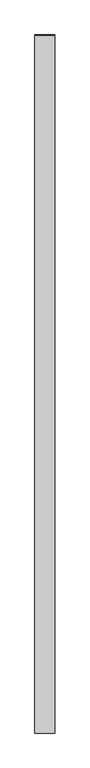
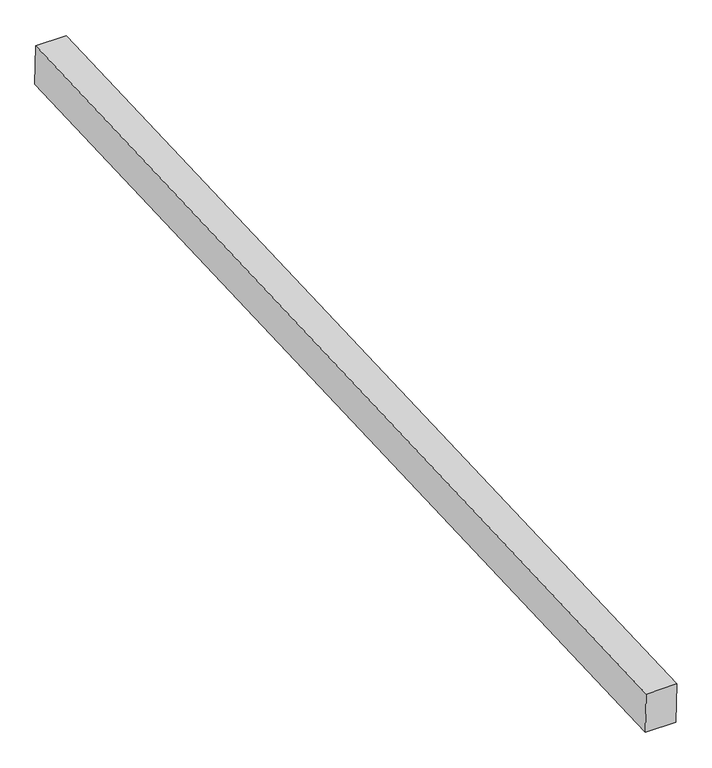
"""IFC4 building model written with IfcOpenShell, lengths in millimetres: proxy geometry, Generic Models 7:Generic Models 1:8:Generic Models 1:8 : Generic Models 7:Generic Models 1:337419:20 : Generic Models 7:Generic Models 1:8:Generic Models 1:8 : Generic Models 7:Generic Models 1:337419:315935."""

from ifc_helpers import new_model, si_unit, frame, origin, place, context, project, spatial, polyline, outline, extrude, source, transform, mapped, element, save


def generic_models_9adc90d8(model_context):
    return source(origin(), model_context, "Body", "SweptSolid", [
        extrude(outline(polyline([(-580626.555738, 3844.0209448), (-575753.6328438, 4047.0593987), (-575746.0659221, 3856.7093942), (-580618.6251193, 3653.6860944), (-580626.555738, 3844.0209448)])), frame((588762.861724, 0.0, 0.0), z_axis=(1.0, 0.0, 0.0), x_axis=(0.0, 1.0, 0.0)), (0.0, 0.0, 1.0), 139.7),
    ])


if __name__ == "__main__":
    model = new_model("IFC4")
    model_context = context("Model", 3, world=origin())
    ifc_project = project(units=[si_unit("LENGTHUNIT", "METRE", prefix="MILLI")], contexts=[model_context])
    site = spatial("IfcSite", under=ifc_project)
    building = spatial("IfcBuilding", under=site)
    placement = place(None, origin())
    generic_models_shape = generic_models_9adc90d8(model_context)
    element("IfcBuildingElementProxy", 1, Name="Generic Models 7:Generic Models 1:8:Generic Models 1:8 : Generic Models 7:Generic Models 1:337419:20 : Generic Models 7:Generic Models 1:8:Generic Models 1:8 : Generic Models 7:Generic Models 1:337419:315935", ObjectType="Generic Models 7:Generic Models 1:8:Generic Models 1:8 : Generic Models 7:Generic Models 1:337419:20 : Generic Models 7:Generic Models 1:8:Generic Models 1:8 : Generic Models 7:Generic Models 1:337419:315935", at=placement, inside=building, context=model_context, shape_type="MappedRepresentation", body=[
        mapped(generic_models_shape, transform((0.0, 0.0, 0.0), x_axis=(1.0, 0.0, 0.0), y_axis=(0.0, 1.0, 0.0), z_axis=(0.0, 0.0, 1.0))),
    ])
    save(model, "model.ifc")

# Revit data of these elements
# Type "Generic Models 7:Generic Models 1:8:Generic Models 1:8 : Generic Models 7:Generic Models 1:337419:20 : Generic Models 7:Generic Models 1:8:Generic Models 1:8 : Generic Models 7:Generic Models 1:337419:315935"
#   NameOverride = "Generic Models 7:Generic Models 1:8:Generic Models 1:8 : Generic Models 7:Generic Models 1:337419:315935"
#   ObjectTypeOverride = "Generic Models 1:8 : Generic Models 7:Generic Models 1:337419"
#   Reference = "Generic Models 1"
#   Tag = "315935"
# Element 1 (IfcBuildingElementProxy, "Generic Models 7:Generic Models 1:8:Generic Models 1:8 : Generic Models 7:Generic Models 1:337419:20 : Generic Models 7:Generic Models 1:8:Generic Models 1:8 : Generic Models 7:Generic Models 1:337419:315935")
#   Materials on its faces: "5 1/2\" X 7 1/2\" EXTERIOR GRADE GLULAM BEAMS"
# Materials
#   "5 1/2\" X 7 1/2\" EXTERIOR GRADE GLULAM BEAMS": class "Wood", colour RGB 183 134 68, transparency 0, Keynote = "M06181300.01", Description = "Pinus Echinata", Cost = 0
